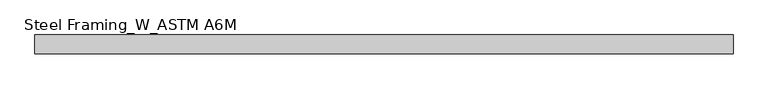
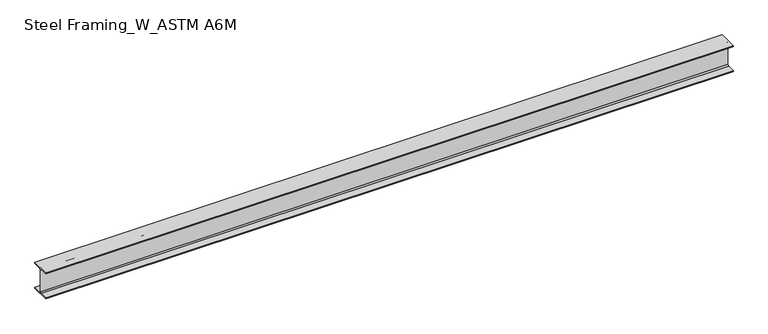
"""IFC4 building model written with IfcOpenShell, lengths in millimetres: beam geometry, Steel Framing_W_ASTM A6M : H_SB_AR_S02_W310x60_G4."""

from ifc_helpers import new_model, si_unit, point, frame, frame_2d, origin, place, context, project, spatial, polyline, circle_curve, trimmed, segment, composite_curve, outline, extrude, source, transform, mapped, element, save


def steel_framing_w_astm_a6m_8cea9429(model_context):
    return source(origin(), model_context, "Body", "SweptSolid", [
        extrude(outline(composite_curve([segment(polyline([(101.5, -137.9), (101.5, -151.0), (-101.5, -151.0), (-101.5, -137.9), (-16.545, -137.9)]), True, "CONTINUOUS"), segment(trimmed(circle_curve(frame_2d((-16.545, -125.1)), 12.8), [point((-16.545, -137.9))], [point((-3.745, -125.1))], True, "CARTESIAN"), True, "CONTINUOUS"), segment(polyline([(-3.745, -125.1), (-3.745, 125.1)]), True, "CONTINUOUS"), segment(trimmed(circle_curve(frame_2d((-16.545, 125.1)), 12.8), [point((-3.745, 125.1))], [point((-16.545, 137.9))], True, "CARTESIAN"), True, "CONTINUOUS"), segment(polyline([(-16.545, 137.9), (-101.5, 137.9), (-101.5, 151.0), (101.5, 151.0), (101.5, 137.9), (16.545, 137.9)]), True, "CONTINUOUS"), segment(trimmed(circle_curve(frame_2d((16.545, 125.1)), 12.8), [point((16.545, 137.9))], [point((3.745, 125.1))], True, "CARTESIAN"), True, "CONTINUOUS"), segment(polyline([(3.745, 125.1), (3.745, -125.1)]), True, "CONTINUOUS"), segment(trimmed(circle_curve(frame_2d((16.545, -125.1)), 12.8), [point((3.745, -125.1))], [point((16.545, -137.9))], True, "CARTESIAN"), True, "CONTINUOUS"), segment(polyline([(16.545, -137.9), (101.5, -137.9)]), True, "CONTINUOUS")], self_intersect=False)), frame((-3753.8, 0.0, 0.0), z_axis=(1.0, 0.0, 0.0), x_axis=(0.0, 1.0, 0.0)), (0.0, 0.0, 1.0), 7507.6),
    ])


if __name__ == "__main__":
    model = new_model("IFC4")
    model_context = context("Model", 3, world=origin())
    ifc_project = project(units=[si_unit("LENGTHUNIT", "METRE", prefix="MILLI")], contexts=[model_context])
    site = spatial("IfcSite", under=ifc_project)
    building = spatial("IfcBuilding", under=site)
    placement = place(None, origin())
    steel_framing_w_astm_a6m_shape = steel_framing_w_astm_a6m_8cea9429(model_context)
    element("IfcBeam", 1, ObjectType="Steel Framing_W_ASTM A6M : H_SB_AR_S02_W310x60_G4", at=placement, inside=building, context=model_context, shape_type="MappedRepresentation", body=[
        mapped(steel_framing_w_astm_a6m_shape, transform((0.0, 0.0, 0.0), x_axis=(1.0, 0.0, 0.0), y_axis=(0.0, 1.0, 0.0), z_axis=(0.0, 0.0, 1.0))),
    ])
    save(model, "model.ifc")

# Revit data of these elements
# Type "Steel Framing_W_ASTM A6M : H_SB_AR_S02_W310x60_G4"
#   Type Mark = "G4"
#   Section Name Key = "W12x40"
#   Width = 20.3 cm
#   Web Thickness = 0.749 cm
#   Web Fillet = 1.28 cm
#   Warping Constant = 387000.0 cm⁶
#   Torsional Moment of Inertia = 37.70 cm⁴
#   Section Area = 75.5 cm²
#   Plastic Modulus weak axis = 275.0 cm³
#   Plastic Modulus strong axis = 934.0 cm³
#   Perimeter = 1.38 m²/m
#   Nominal Weight = 60.00 kgf/m
#   Moment of Inertia weak axis = 1840.00 cm⁴
#   Moment of Inertia strong axis = 12800.00 cm⁴
#   Height = 30.2 cm
#   Flange Thickness = 1.31 cm
#   Elastic Modulus weak axis = 180.0 cm³
#   Elastic Modulus strong axis = 844.0 cm³
#   Centroid Vertical = 15.1 cm
#   Centroid Horizontal = 10.15 cm
#   Length [instance default] = 1500 mm
#   Structural Material [instance default] = Steel, 45-345
#   Bolt Spacing = 0
#   Assembly Code = ""
# Element 1 (IfcBeam, "Steel Framing_W_ASTM A6M : H_SB_AR_S02_W310x60_G4")
#   Materials on its faces: "Steel, 45-345"
# Materials
#   "Steel, 45-345": class "Metal", colour RGB 189 187 185, transparency 0, Description = "Steel 345 MPa", Cost = 0
